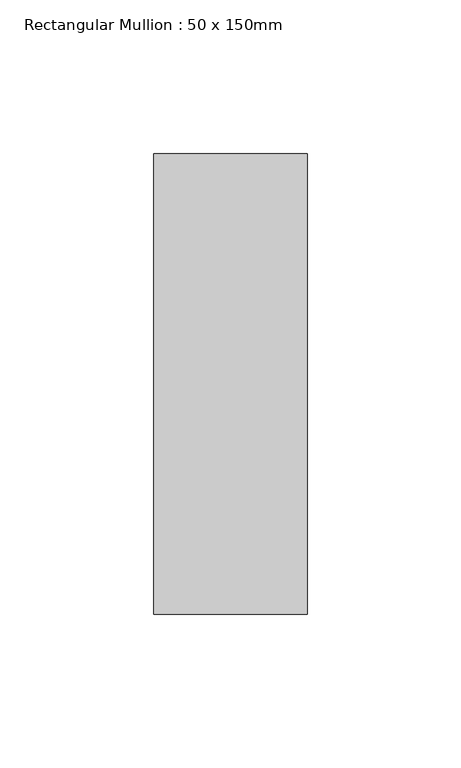
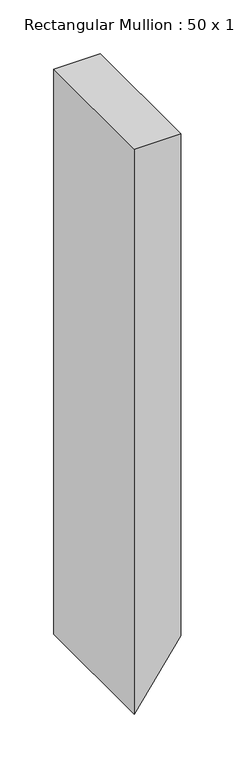
"""IFC4 building model written with IfcOpenShell, lengths in millimetres: member geometry, Rectangular Mullion : 50 x 150mm."""

from ifc_helpers import new_model, si_unit, frame, origin, place, context, project, spatial, polyline, outline, extrude, source, transform, mapped, element, save


def rectangular_mullion_50_x_150mm_15015eac(model_context):
    return source(origin(), model_context, "Body", "SweptSolid", [
        extrude(outline(polyline([(0.0, 25.0), (0.0, -25.0), (-641.6425563, -25.0), (-570.235156, 25.0), (0.0, 25.0)])), frame((0.0, -75.0, 0.0), z_axis=(0.0, 1.0, 0.0), x_axis=(0.0, 0.0, 1.0)), (0.0, 0.0, 1.0), 150.0),
    ])


if __name__ == "__main__":
    model = new_model("IFC4")
    model_context = context("Model", 3, world=origin())
    ifc_project = project(units=[si_unit("LENGTHUNIT", "METRE", prefix="MILLI")], contexts=[model_context])
    site = spatial("IfcSite", under=ifc_project)
    building = spatial("IfcBuilding", under=site)
    placement = place(None, origin())
    rectangular_mullion_50_x_150mm_shape = rectangular_mullion_50_x_150mm_15015eac(model_context)
    element("IfcMember", 1, ObjectType="Rectangular Mullion : 50 x 150mm", at=placement, inside=building, context=model_context, shape_type="MappedRepresentation", body=[
        mapped(rectangular_mullion_50_x_150mm_shape, transform((0.0, 0.0, 0.0), x_axis=(1.0, 0.0, 0.0), y_axis=(0.0, 1.0, 0.0), z_axis=(0.0, 0.0, 1.0))),
    ])
    save(model, "model.ifc")

# Revit data of these elements
# Type "Rectangular Mullion : 50 x 150mm"
#   built-in parameter 1007304 = 0.492126 (stored number, unit not read)
#   built-in parameter 1007301 = 0.082021 (stored number, unit not read)
#   built-in parameter 1007300 = 0.082021 (stored number, unit not read)
# Element 1 (IfcMember, "Rectangular Mullion : 50 x 150mm")
#   Materials on its faces: "Aluminium"
# Materials
#   "Aluminium": class "Metal", colour RGB 247 247 247, transparency 0, Description = "Aluminium 6061", Cost = 0
